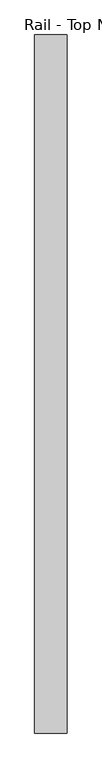
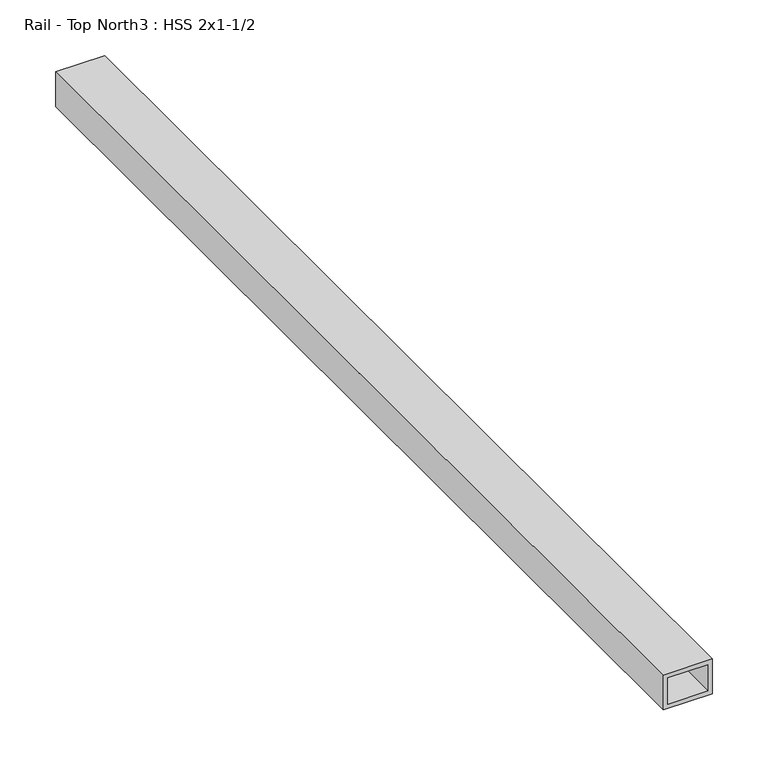
"""IFC4 building model written with IfcOpenShell, lengths in millimetres: proxy geometry, Rail - Top North3 : HSS 2x1-1/2."""

from ifc_helpers import new_model, si_unit, frame, origin, place, context, project, spatial, polyline, outline, extrude, source, transform, mapped, element, save


def rail_top_north3_hss_2x1_1_2_5f745a76(model_context):
    return source(origin(), model_context, "Body", "SweptSolid", [
        extrude(outline(polyline([(2400.3, 587416.6934739), (2438.4, 587416.6934739), (2438.4, 587365.8934739), (2400.3, 587365.8934739), (2400.3, 587416.6934739)]), holes=[polyline([(2433.6375, 587411.9309739), (2405.0625, 587411.9309739), (2405.0625, 587370.6559739), (2433.6375, 587370.6559739), (2433.6375, 587411.9309739)])]), frame((0.0, -535201.5663841, 0.0), z_axis=(0.0, 1.0, 0.0), x_axis=(0.0, 0.0, 1.0)), (0.0, 0.0, 1.0), 1092.2),
    ])


if __name__ == "__main__":
    model = new_model("IFC4")
    model_context = context("Model", 3, world=origin())
    ifc_project = project(units=[si_unit("LENGTHUNIT", "METRE", prefix="MILLI")], contexts=[model_context])
    site = spatial("IfcSite", under=ifc_project)
    building = spatial("IfcBuilding", under=site)
    placement = place(None, origin())
    rail_top_north3_hss_2x1_1_2_shape = rail_top_north3_hss_2x1_1_2_5f745a76(model_context)
    element("IfcBuildingElementProxy", 1, Name="Rail - Top North3 : HSS 2x1-1/2", ObjectType="Rail - Top North3 : HSS 2x1-1/2", at=placement, inside=building, context=model_context, shape_type="MappedRepresentation", body=[
        mapped(rail_top_north3_hss_2x1_1_2_shape, transform((0.0, 0.0, 0.0), x_axis=(1.0, 0.0, 0.0), y_axis=(0.0, 1.0, 0.0), z_axis=(0.0, 0.0, 1.0))),
    ])
    save(model, "model.ifc")

# Revit data of these elements
# Element 1 (IfcBuildingElementProxy, "Rail - Top North3 : HSS 2x1-1/2")
#   Materials on its faces: "1-1/2\"X2\" GALV. STL HSS TUBING"
# Materials
#   "1-1/2\"X2\" GALV. STL HSS TUBING": class "Generic", colour RGB 211 211 207, transparency 0, Cost = 0
